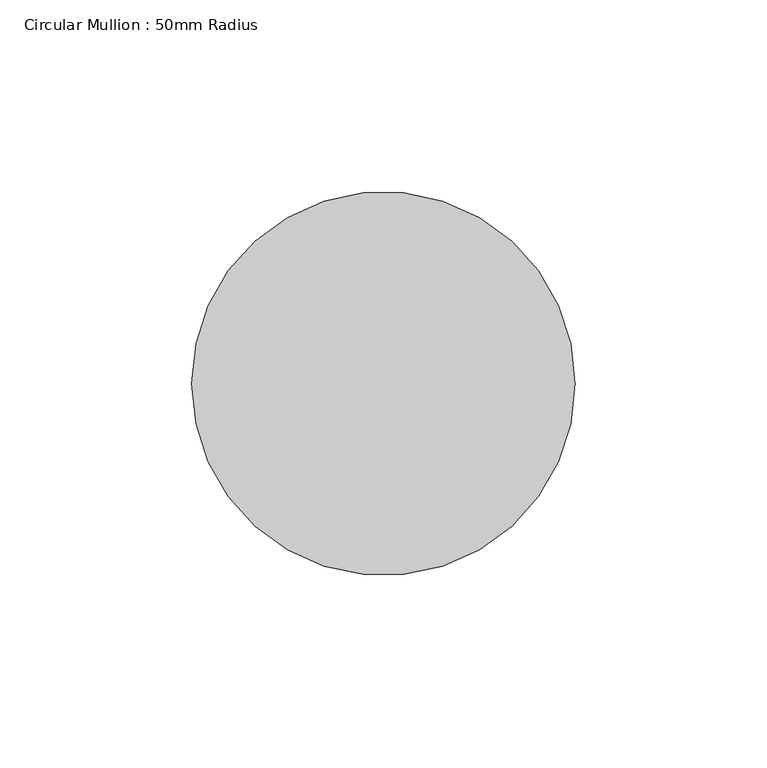
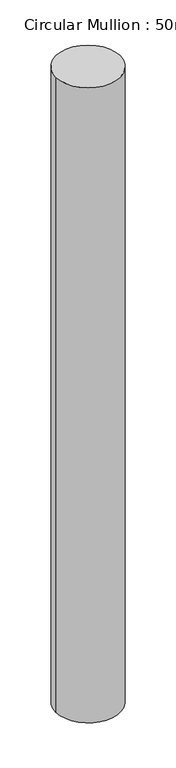
"""IFC4 building model written with IfcOpenShell, lengths in millimetres: member geometry, Circular Mullion : 50mm Radius."""

from ifc_helpers import new_model, si_unit, point, frame, origin, origin_2d, place, context, project, spatial, circle_curve, trimmed, segment, composite_curve, outline, extrude, source, transform, mapped, element, save


def circular_mullion_50mm_radius_9a90d978(model_context):
    return source(origin(), model_context, "Body", "SweptSolid", [
        extrude(outline(composite_curve([segment(trimmed(circle_curve(origin_2d(), 50.0), [point((50.0, 0.0))], [point((-50.0, 0.0))], False, "CARTESIAN"), True, "CONTINUOUS"), segment(trimmed(circle_curve(origin_2d(), 50.0), [point((-50.0, 0.0))], [point((50.0, 0.0))], False, "CARTESIAN"), True, "CONTINUOUS")], self_intersect=False)), frame((0.0, 0.0, -1039.1222403), z_axis=(0.0, 0.0, 1.0), x_axis=(1.0, 0.0, 0.0)), (0.0, 0.0, 1.0), 1039.1222403),
    ])


if __name__ == "__main__":
    model = new_model("IFC4")
    model_context = context("Model", 3, world=origin())
    ifc_project = project(units=[si_unit("LENGTHUNIT", "METRE", prefix="MILLI")], contexts=[model_context])
    site = spatial("IfcSite", under=ifc_project)
    building = spatial("IfcBuilding", under=site)
    placement = place(None, origin())
    circular_mullion_50mm_radius_shape = circular_mullion_50mm_radius_9a90d978(model_context)
    element("IfcMember", 1, ObjectType="Circular Mullion : 50mm Radius", at=placement, inside=building, context=model_context, shape_type="MappedRepresentation", body=[
        mapped(circular_mullion_50mm_radius_shape, transform((0.0, 0.0, 0.0), x_axis=(1.0, 0.0, 0.0), y_axis=(0.0, 1.0, 0.0), z_axis=(0.0, 0.0, 1.0))),
    ])
    save(model, "model.ifc")

# Revit data of these elements
# Type "Circular Mullion : 50mm Radius"
#   built-in parameter 1007350 = 0.164042 (stored number, unit not read)
# Element 1 (IfcMember, "Circular Mullion : 50mm Radius")
#   Materials on its faces: "Aluminium"
# Materials
#   "Aluminium": class "Metal", colour RGB 247 247 247, transparency 0, Description = "Aluminium 6061", Cost = 0
